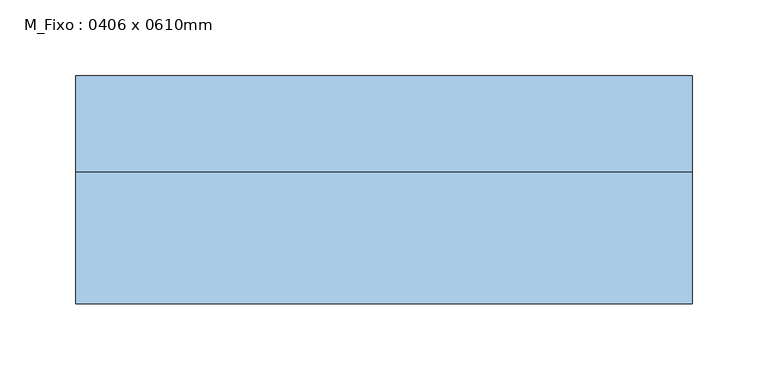
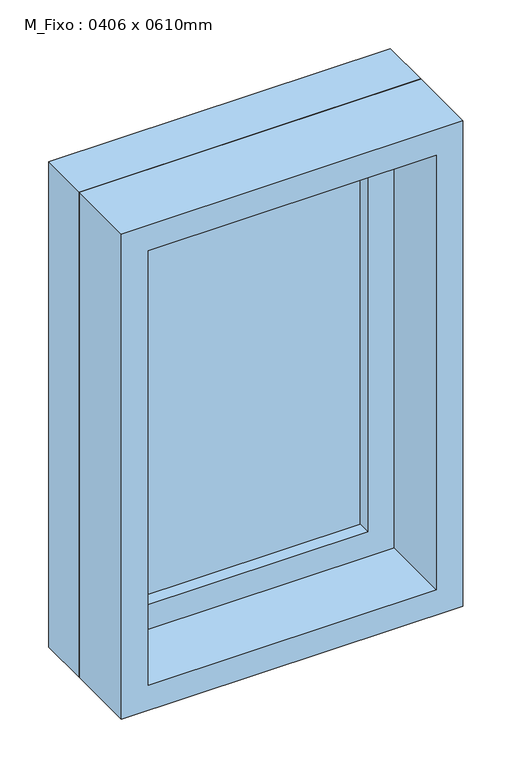
"""IFC4 building model written with IfcOpenShell, lengths in millimetres: window geometry, M_Fixo : 0406 x 0610mm."""

import ifcopenshell
import ifcopenshell.guid

model = None  # the IFC model being written
_history = None  # IfcOwnerHistory: only IFC2X3 demands one
_inside = {}  # id of a spatial element -> (the spatial element, [elements in it])
_under = {}  # id of a project, library or spatial element -> (it, [spatial elements below it])
_declared = {}  # id of a project -> (the project, [libraries it declares])
_typed = {}  # id of a type object -> (the type object, [elements of that type])
_made_of = {}  # id of a material, layer set ... -> (it, [elements and type objects made of it])


def new_model(schema):
    """Start an empty IFC model of exactly this schema.

    Asked for "IFC4X3", IfcOpenShell would pick the latest addendum, in which some entities
    have other attributes; the version numbers below select the first issue.
    IFC2X3 requires an IfcOwnerHistory on every rooted entity: one is made here for all.
    """
    global model, _history
    if schema == "IFC4X3":
        model = ifcopenshell.file(schema_version=(4, 3, 0, 0))
    else:
        model = ifcopenshell.file(schema=schema)
    _inside.clear()
    _under.clear()
    _declared.clear()
    _typed.clear()
    _made_of.clear()
    _history = None
    if model.schema == "IFC2X3":
        org = make("IfcOrganization", Name="unknown")
        user = make(
            "IfcPersonAndOrganization",
            ThePerson=make("IfcPerson", FamilyName="unknown"),
            TheOrganization=org,
        )
        app = make(
            "IfcApplication",
            ApplicationDeveloper=org,
            Version="unknown",
            ApplicationFullName="unknown",
            ApplicationIdentifier="unknown",
        )
        _history = make(
            "IfcOwnerHistory",
            OwningUser=user,
            OwningApplication=app,
            ChangeAction="ADDED",
            CreationDate=0,
        )
    return model


def make(cls, **values):
    """One entity of the class cls with the attributes given. An attribute that is None is left unset."""
    return model.create_entity(
        cls, **{name: value for name, value in values.items() if value is not None}
    )


def rooted(cls, **values):
    """An entity with a GlobalId (a new one), such as an element, a storey or a relation."""
    return make(cls, GlobalId=ifcopenshell.guid.new(), OwnerHistory=_history, **values)


def si_unit(unit_type, name, prefix=None):
    """IfcSIUnit, for example si_unit("LENGTHUNIT", "METRE", prefix="MILLI")."""
    return make("IfcSIUnit", UnitType=unit_type, Prefix=prefix, Name=name)


def assignment(units):
    """IfcUnitAssignment: the units of a project."""
    return None if units is None else make("IfcUnitAssignment", Units=units)


def point(xyz):
    """IfcCartesianPoint."""
    return None if xyz is None else make("IfcCartesianPoint", Coordinates=xyz)


def direction(xyz):
    """IfcDirection."""
    return None if xyz is None else make("IfcDirection", DirectionRatios=xyz)


def frame(location, z_axis=None, x_axis=None):
    """IfcAxis2Placement3D, a coordinate frame: its origin and axes. An axis left out is left unset."""
    return make(
        "IfcAxis2Placement3D",
        Location=point(location),
        Axis=direction(z_axis),
        RefDirection=direction(x_axis),
    )


def origin():
    """The frame at (0, 0, 0) with its axes left unset."""
    return frame((0.0, 0.0, 0.0))


def place(relative_to, where):
    """IfcLocalPlacement: puts the frame where relative to a parent placement (None: the world)."""
    return make(
        "IfcLocalPlacement", PlacementRelTo=relative_to, RelativePlacement=where
    )


def context(
    kind, dimensions, precision=None, world=None, true_north=None, identifier=None
):
    """IfcGeometricRepresentationContext, for example the 3D "Model" context."""
    return make(
        "IfcGeometricRepresentationContext",
        ContextIdentifier=identifier,
        ContextType=kind,
        CoordinateSpaceDimension=dimensions,
        Precision=precision,
        WorldCoordinateSystem=world,
        TrueNorth=true_north,
    )


def project(units=None, contexts=None):
    """IfcProject with its units and contexts."""
    return rooted(
        "IfcProject",
        Name="project",
        RepresentationContexts=contexts,
        UnitsInContext=assignment(units),
    )


def spatial(cls, under=None, at=None, **own):
    """A site, building, storey or space (cls), placed at a placement, below another one or the project."""
    s = rooted(cls, ObjectPlacement=at, **own)
    if under is not None:
        _under.setdefault(under.id(), (under, []))[1].append(s)
    return s


def polyline(points):
    """IfcPolyline through the points."""
    return make("IfcPolyline", Points=[point(p) for p in points])


def outline(outer, holes=None, kind="AREA"):
    """IfcArbitraryClosedProfileDef: a profile drawn as a closed curve; with holes, ...WithVoids."""
    if holes is None:
        return make("IfcArbitraryClosedProfileDef", ProfileType=kind, OuterCurve=outer)
    return make(
        "IfcArbitraryProfileDefWithVoids",
        ProfileType=kind,
        OuterCurve=outer,
        InnerCurves=holes,
    )


def extrude(swept, where, along, depth):
    """IfcExtrudedAreaSolid: the profile swept, set in the frame where, extruded along a direction by depth."""
    return make(
        "IfcExtrudedAreaSolid",
        SweptArea=swept,
        Position=where,
        ExtrudedDirection=direction(along),
        Depth=depth,
    )


def shape(context_of_items, identifier, shape_type, items):
    """IfcShapeRepresentation: the items that make up one representation, for example the "Body"."""
    return make(
        "IfcShapeRepresentation",
        ContextOfItems=context_of_items,
        RepresentationIdentifier=identifier,
        RepresentationType=shape_type,
        Items=items,
    )


def source(mapping_origin, context_of_items, identifier, shape_type, items):
    """IfcRepresentationMap: a shape defined once, which mapped items show again and again."""
    return make(
        "IfcRepresentationMap",
        MappingOrigin=mapping_origin,
        MappedRepresentation=shape(context_of_items, identifier, shape_type, items),
    )


def transform(
    local_origin,
    x_axis=None,
    y_axis=None,
    z_axis=None,
    scale=None,
    scale2=None,
    scale3=None,
    uniform=True,
):
    """IfcCartesianTransformationOperator3D, or its non-uniform kind. x_axis, y_axis, z_axis: its Axis1, 2, 3."""
    if uniform:
        return make(
            "IfcCartesianTransformationOperator3D",
            Axis1=direction(x_axis),
            Axis2=direction(y_axis),
            LocalOrigin=point(local_origin),
            Scale=scale,
            Axis3=direction(z_axis),
        )
    return make(
        "IfcCartesianTransformationOperator3DnonUniform",
        Axis1=direction(x_axis),
        Axis2=direction(y_axis),
        LocalOrigin=point(local_origin),
        Scale=scale,
        Axis3=direction(z_axis),
        Scale2=scale2,
        Scale3=scale3,
    )


def mapped(mapping_source, mapping_target):
    """IfcMappedItem: shows the shape of a source again, moved by a transform."""
    return make(
        "IfcMappedItem", MappingSource=mapping_source, MappingTarget=mapping_target
    )


def made_of(thing, what):
    """Note that an element or type object is made of a material, layer set ...; save() writes the relation."""
    if what is not None:
        _made_of.setdefault(what.id(), (what, []))[1].append(thing)
    return thing


def element(
    cls,
    number,
    at=None,
    inside=None,
    cuts=None,
    type_object=None,
    material=None,
    context=None,
    identifier="Body",
    shape_type=None,
    held_by="IfcProductDefinitionShape",
    body=None,
    shapes=None,
    **own,
):
    """One element of the class cls, such as IfcWall. Its Tag is "e" and its number.

    at: its placement. inside: the storey or other place that contains it. cuts: it is an
    opening in that element (IfcRelVoidsElement). A single representation is given by context,
    identifier, shape_type and body (its items); several are given by shapes. held_by: the class
    of the entity that holds the representations. save() writes the other relations.
    """
    e = rooted(cls, Tag="e%d" % number, ObjectPlacement=at, **own)
    if body is not None:
        shapes = [shape(context, identifier, shape_type, body)]
    if shapes is not None:
        e.Representation = make(held_by, Representations=shapes)
    if inside is not None:
        _inside.setdefault(inside.id(), (inside, []))[1].append(e)
    if cuts is not None:
        rooted(
            "IfcRelVoidsElement", RelatingBuildingElement=cuts, RelatedOpeningElement=e
        )
    if type_object is not None:
        _typed.setdefault(type_object.id(), (type_object, []))[1].append(e)
    return made_of(e, material)


def aggregate(whole, parts):
    """IfcRelAggregates: a whole, such as a stair, and the parts it consists of."""
    return rooted("IfcRelAggregates", RelatingObject=whole, RelatedObjects=parts)


def save(model, path):
    """Write the relations noted so far, then the file.

    IfcRelAggregates (storeys below a building ...), IfcRelContainedInSpatialStructure (elements
    in a storey), IfcRelDefinesByType, IfcRelAssociatesMaterial and IfcRelDeclares: one each for
    every whole, place, type object, material and project.
    """
    for whole, parts in _under.values():
        aggregate(whole, parts)
    for where, things in _inside.values():
        rooted(
            "IfcRelContainedInSpatialStructure",
            RelatedElements=things,
            RelatingStructure=where,
        )
    for kind, things in _typed.values():
        rooted("IfcRelDefinesByType", RelatedObjects=things, RelatingType=kind)
    for what, things in _made_of.values():
        rooted("IfcRelAssociatesMaterial", RelatedObjects=things, RelatingMaterial=what)
    for by, libraries in _declared.values():
        rooted("IfcRelDeclares", RelatingContext=by, RelatedDefinitions=libraries)
    model.write(path)


def m_fixo_0406_x_0610mm_893b2dd9(model_context):
    return source(origin(), model_context, "Body", "SweptSolid", [
        extrude(outline(polyline([(-140.0, 53.0), (140.0, 53.0), (140.0, 41.0), (-140.0, 41.0), (-140.0, 53.0)])), frame((0.0, 0.0, 978.0), z_axis=(0.0, 0.0, 1.0), x_axis=(1.0, 0.0, 0.0)), (0.0, 0.0, 1.0), 484.0),
        extrude(outline(polyline([(1506.0, -184.0), (934.0, -184.0), (934.0, 184.0), (1506.0, 184.0), (1506.0, -184.0)]), holes=[polyline([(1462.0, -140.0), (1462.0, 140.0), (978.0, 140.0), (978.0, -140.0), (1462.0, -140.0)])]), frame((0.0, 25.0, 0.0), z_axis=(0.0, 1.0, 0.0), x_axis=(0.0, 0.0, 1.0)), (0.0, 0.0, 1.0), 44.0),
        extrude(outline(polyline([(1525.0, -203.0), (915.0, -203.0), (915.0, 203.0), (1525.0, 203.0), (1525.0, -203.0)]), holes=[polyline([(1506.0, -184.0), (1506.0, 184.0), (934.0, 184.0), (934.0, -184.0), (1506.0, -184.0)])]), frame((0.0, 25.0, 0.0), z_axis=(0.0, 1.0, 0.0), x_axis=(0.0, 0.0, 1.0)), (0.0, 0.0, 1.0), 63.0),
        extrude(outline(polyline([(1525.0, -203.0), (915.0, -203.0), (915.0, 203.0), (1525.0, 203.0), (1525.0, -203.0)]), holes=[polyline([(1493.0, -171.0), (1493.0, 171.0), (947.0, 171.0), (947.0, -171.0), (1493.0, -171.0)])]), frame((0.0, -62.0, 0.0), z_axis=(0.0, 1.0, 0.0), x_axis=(0.0, 0.0, 1.0)), (0.0, 0.0, 1.0), 87.0),
    ])


if __name__ == "__main__":
    model = new_model("IFC4")
    model_context = context("Model", 3, world=origin())
    ifc_project = project(units=[si_unit("LENGTHUNIT", "METRE", prefix="MILLI")], contexts=[model_context])
    site = spatial("IfcSite", under=ifc_project)
    building = spatial("IfcBuilding", under=site)
    placement = place(None, origin())
    m_fixo_0406_x_0610mm_shape = m_fixo_0406_x_0610mm_893b2dd9(model_context)
    element("IfcWindow", 1, ObjectType="M_Fixo : 0406 x 0610mm", at=placement, inside=building, context=model_context, shape_type="MappedRepresentation", body=[
        mapped(m_fixo_0406_x_0610mm_shape, transform((0.0, 0.0, 0.0), x_axis=(1.0, 0.0, 0.0), y_axis=(0.0, 1.0, 0.0), z_axis=(0.0, 0.0, 1.0))),
    ])
    save(model, "model.ifc")

# Revit data of these elements
# Type "M_Fixo : 0406 x 0610mm"
#   Type Mark = "10"
#   Construction Type Id = "GSP4R"
#   Analytic Construction = "Vidraça única Pilkington 1/8 pol"
#   Visual Light Transmittance = 0.9
#   Thermal Resistance (R) = 0.271106 (m²·K)/W
#   Solar Heat Gain Coefficient = 0.78
#   Heat Transfer Coefficient (U) = 3.6886 W/(m²·K)
#   Height = 0.61 m
#   Altura-padrão do peitoril = 0.915 m
#   Width = 0.406 m
#   Janela aplicada = 0.019 m
#   Material da estrutura externa = Caixilho
#   Material da estrutura interna = Caixilho
#   Material do painel de vidro = Vidro
#   Caixilho = Caixilho
#   Wall Closure = (empty or 0)
# Element 1 (IfcWindow, "M_Fixo : 0406 x 0610mm")
#   Materials on its faces: "Caixilho", "Vidro"
# Materials
#   "Caixilho": class "Madeira", colour RGB 224 178 126, transparency 0, Cost = 0
#   "Vidro": class "Vidro", colour RGB 0 128 192, transparency 0.9, Description = "Vidro de sílica", Cost = 0
